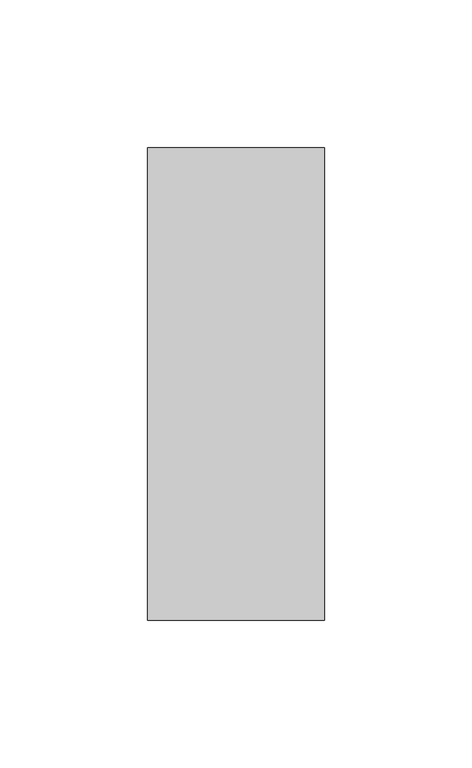
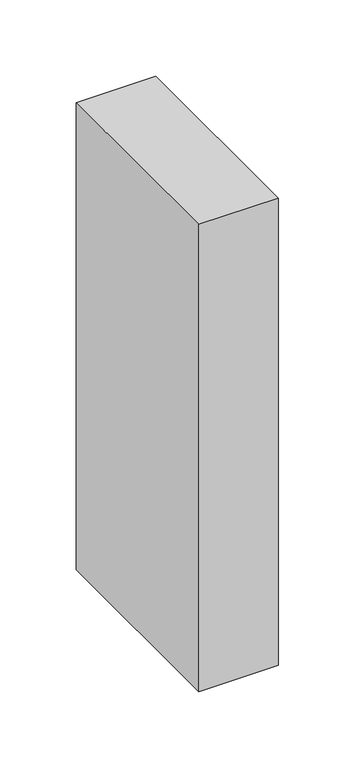
"""IFC4 building model written with IfcOpenShell, lengths in millimetres: column geometry, Madeira de lei-Coluna : Pontalete 6X16cm."""

from ifc_helpers import new_model, si_unit, frame, origin, place, context, project, spatial, polyline, outline, extrude, source, transform, mapped, element, save


def column_c7348c99(model_context):
    return source(origin(), model_context, "Body", "SweptSolid", [
        extrude(outline(polyline([(30.0, 80.0), (30.0, -80.0), (-30.0, -80.0), (-30.0, 80.0), (30.0, 80.0)])), frame((0.0, 0.0, 4460.0), z_axis=(0.0, 0.0, 1.0), x_axis=(1.0, 0.0, 0.0)), (0.0, 0.0, 1.0), 372.8),
    ])


if __name__ == "__main__":
    model = new_model("IFC4")
    model_context = context("Model", 3, world=origin())
    ifc_project = project(units=[si_unit("LENGTHUNIT", "METRE", prefix="MILLI")], contexts=[model_context])
    site = spatial("IfcSite", under=ifc_project)
    building = spatial("IfcBuilding", under=site)
    placement = place(None, origin())
    column_shape = column_c7348c99(model_context)
    element("IfcColumn", 1, ObjectType="Madeira de lei-Coluna : Pontalete 6X16cm", at=placement, inside=building, context=model_context, shape_type="MappedRepresentation", body=[
        mapped(column_shape, transform((0.0, 0.0, 0.0), x_axis=(1.0, 0.0, 0.0), y_axis=(0.0, 1.0, 0.0), z_axis=(0.0, 0.0, 1.0))),
    ])
    save(model, "model.ifc")

# Revit data of these elements
# Type "Madeira de lei-Coluna : Pontalete 6X16cm"
#   A = 0.01952 m²
#   b = 0.06 m
#   d = 0.16 m
#   Structural Material [instance default] = none
#   Assembly Code = ""
# Element 1 (IfcColumn, "Madeira de lei-Coluna : Pontalete 6X16cm")
#   Structural Material = .MADEIRAMENTO
#   Materials on its faces: ".MADEIRAMENTO"
# Materials
#   ".MADEIRAMENTO": class ".CC_MADEIRAS", colour RGB 212 179 113, transparency 0, Cost = 0
